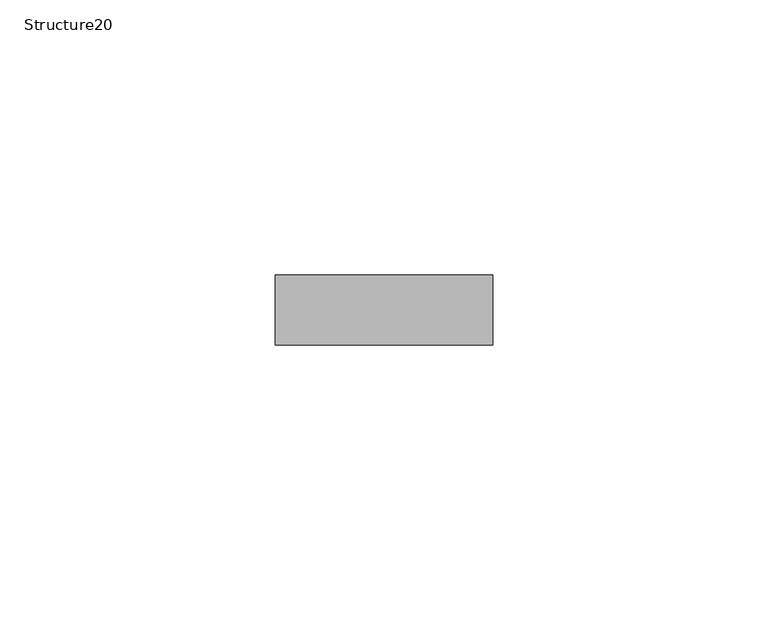
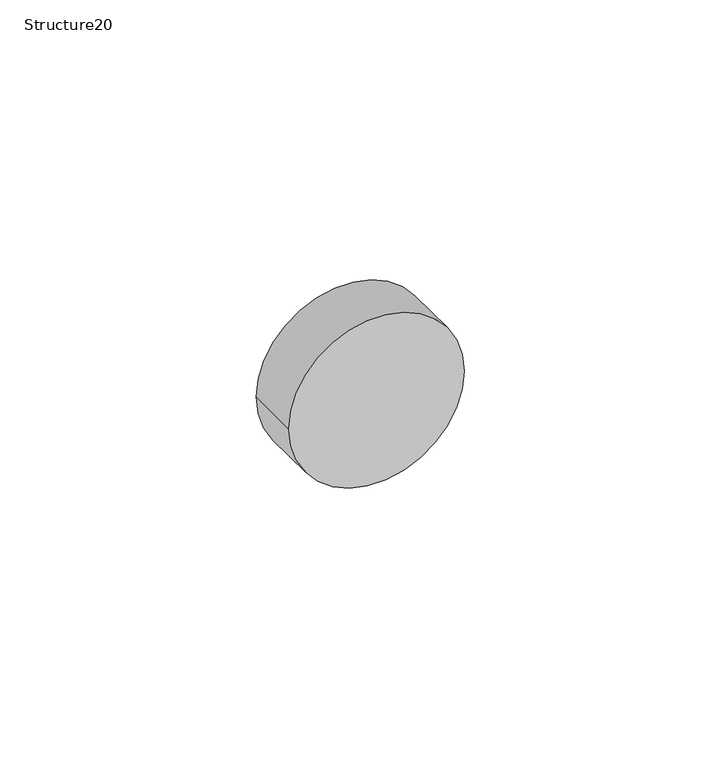
"""IFC4 building model written with IfcOpenShell, lengths in millimetres: proxy geometry, Structure20 : Structure668217148."""

from ifc_helpers import new_model, si_unit, point, frame, frame_2d, origin, place, context, project, spatial, circle_curve, trimmed, segment, composite_curve, outline, extrude, source, transform, mapped, element, save


def structure20_0f52bea8(model_context):
    return source(origin(), model_context, "Body", "SweptSolid", [
        extrude(outline(composite_curve([segment(trimmed(circle_curve(frame_2d((40908.7088339, 9847.8795269)), 19.7708678), [point((40908.7088339, 9828.1086591))], [point((40908.7088339, 9867.6503947))], False, "CARTESIAN"), True, "CONTINUOUS"), segment(trimmed(circle_curve(frame_2d((40908.7088339, 9847.8795269)), 19.7708678), [point((40908.7088339, 9867.6503947))], [point((40908.7088339, 9828.1086591))], False, "CARTESIAN"), True, "CONTINUOUS")], self_intersect=False)), frame((0.0, 1913.4573723, 0.0), z_axis=(0.0, 1.0, 0.0), x_axis=(0.0, 0.0, 1.0)), (0.0, 0.0, 1.0), 12.7),
    ])


if __name__ == "__main__":
    model = new_model("IFC4")
    model_context = context("Model", 3, world=origin())
    ifc_project = project(units=[si_unit("LENGTHUNIT", "METRE", prefix="MILLI")], contexts=[model_context])
    site = spatial("IfcSite", under=ifc_project)
    building = spatial("IfcBuilding", under=site)
    placement = place(None, origin())
    structure20_shape = structure20_0f52bea8(model_context)
    element("IfcBuildingElementProxy", 1, Name="Structure20 : Structure668217148", ObjectType="Structure20 : Structure668217148", at=placement, inside=building, context=model_context, shape_type="MappedRepresentation", body=[
        mapped(structure20_shape, transform((0.0, 0.0, 0.0), x_axis=(1.0, 0.0, 0.0), y_axis=(0.0, 1.0, 0.0), z_axis=(0.0, 0.0, 1.0))),
    ])
    save(model, "model.ifc")

# Revit data of these elements
# Type "Structure20 : Structure668217148"
#   NameOverride = "Structure668217148"
# Element 1 (IfcBuildingElementProxy, "Structure20 : Structure668217148")
#   Materials on its faces: "1.5\" DIA. STAINLESS STEEL RAILING"
# Materials
#   "1.5\" DIA. STAINLESS STEEL RAILING": class "Unassigned", colour RGB 128 128 128, transparency 0, Cost = 0
